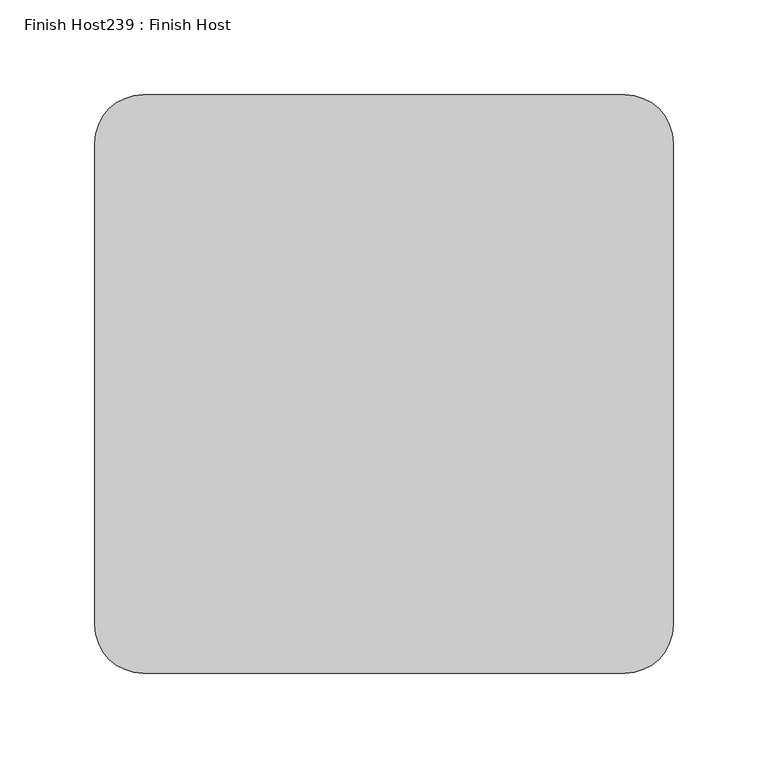
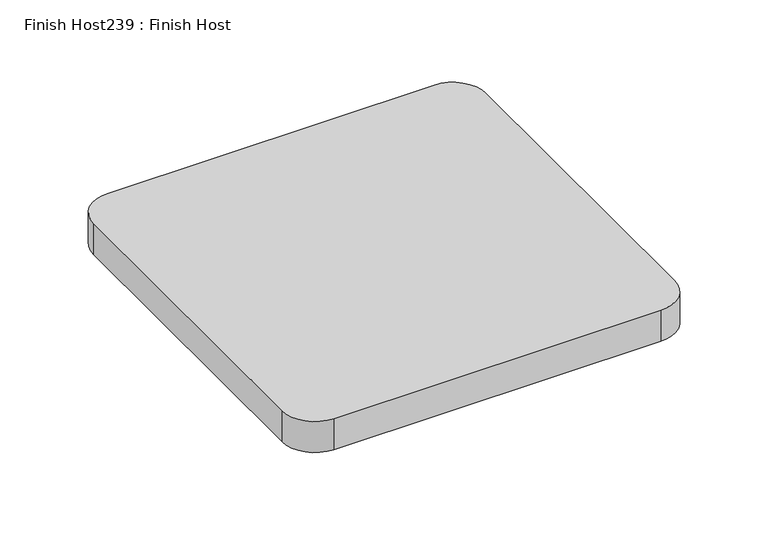
"""IFC4 building model written with IfcOpenShell, lengths in millimetres: proxy geometry, Finish Host239 : Finish Host."""

from ifc_helpers import new_model, si_unit, point, frame_2d, origin, origin_with_axes, place, context, project, spatial, polyline, circle_curve, trimmed, segment, composite_curve, outline, extrude, source, transform, mapped, element, save


def finish_host239_finish_host_ec17311e(model_context):
    return source(origin(), model_context, "Body", "SweptSolid", [
        extrude(outline(composite_curve([segment(polyline([(-886.9269864, 6259.9047826), (-886.9269864, 6513.9047826)]), True, "CONTINUOUS"), segment(trimmed(circle_curve(frame_2d((-861.5269864, 6513.9047826)), 25.4), [point((-886.9269864, 6513.9047826))], [point((-861.5269864, 6539.3047826))], False, "CARTESIAN"), True, "CONTINUOUS"), segment(polyline([(-861.5269864, 6539.3047826), (-607.5269864, 6539.3047826)]), True, "CONTINUOUS"), segment(trimmed(circle_curve(frame_2d((-607.5269864, 6513.9047826)), 25.4), [point((-607.5269864, 6539.3047826))], [point((-582.1269864, 6513.9047826))], False, "CARTESIAN"), True, "CONTINUOUS"), segment(polyline([(-582.1269864, 6513.9047826), (-582.1269864, 6259.9047826)]), True, "CONTINUOUS"), segment(trimmed(circle_curve(frame_2d((-607.5269864, 6259.9047826)), 25.4), [point((-582.1269864, 6259.9047826))], [point((-607.5269864, 6234.5047826))], False, "CARTESIAN"), True, "CONTINUOUS"), segment(polyline([(-607.5269864, 6234.5047826), (-861.5269864, 6234.5047826)]), True, "CONTINUOUS"), segment(trimmed(circle_curve(frame_2d((-861.5269864, 6259.9047826)), 25.4), [point((-861.5269864, 6234.5047826))], [point((-886.9269864, 6259.9047826))], False, "CARTESIAN"), True, "CONTINUOUS")], self_intersect=False)), origin_with_axes(), (0.0, 0.0, 1.0), 25.4),
    ])


if __name__ == "__main__":
    model = new_model("IFC4")
    model_context = context("Model", 3, world=origin())
    ifc_project = project(units=[si_unit("LENGTHUNIT", "METRE", prefix="MILLI")], contexts=[model_context])
    site = spatial("IfcSite", under=ifc_project)
    building = spatial("IfcBuilding", under=site)
    placement = place(None, origin())
    finish_host239_finish_host_shape = finish_host239_finish_host_ec17311e(model_context)
    element("IfcBuildingElementProxy", 1, Name="Finish Host239 : Finish Host", ObjectType="Finish Host239 : Finish Host", at=placement, inside=building, context=model_context, shape_type="MappedRepresentation", body=[
        mapped(finish_host239_finish_host_shape, transform((0.0, 0.0, 0.0), x_axis=(1.0, 0.0, 0.0), y_axis=(0.0, 1.0, 0.0), z_axis=(0.0, 0.0, 1.0))),
    ])
    save(model, "model.ifc")

# Revit data of these elements
# Type "Finish Host239 : Finish Host"
#   Panel Material = Fabric - Teknion - P401 - Peru - Tacna
# Element 1 (IfcBuildingElementProxy, "Finish Host239 : Finish Host")
#   Materials on its faces: "Fabric - Teknion - P401 - Peru - Tacna"
# Materials
#   "Fabric - Teknion - P401 - Peru - Tacna": class "Fabric", colour RGB 62 61 60, transparency 0, Model = "P401", Manufacturer = "Teknion Studio", URL = "http://www.teknionstudio.com/", Description = "Tacna Peru", Cost = 0
